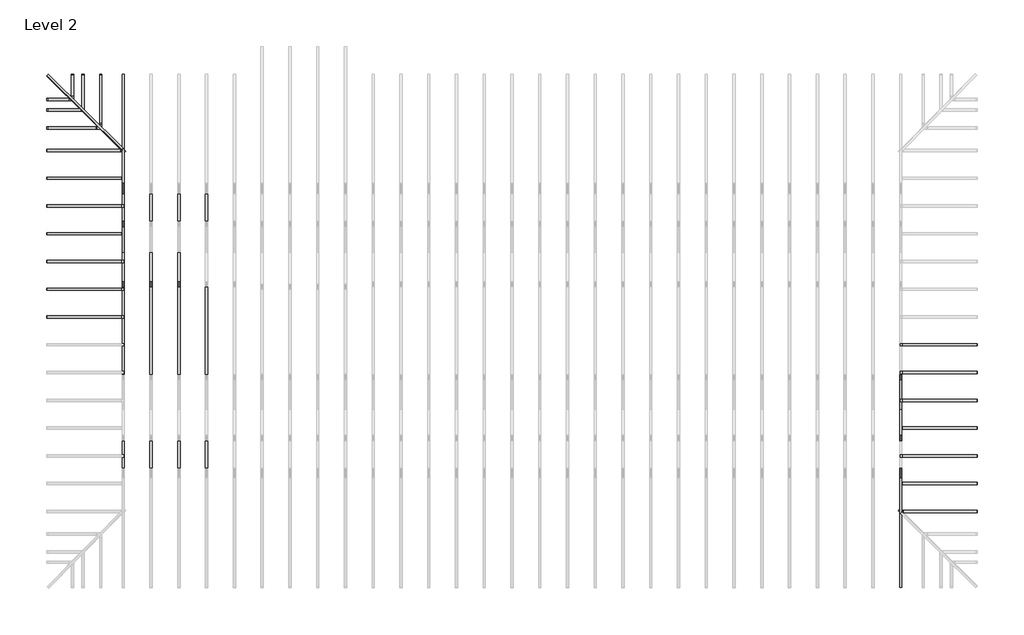
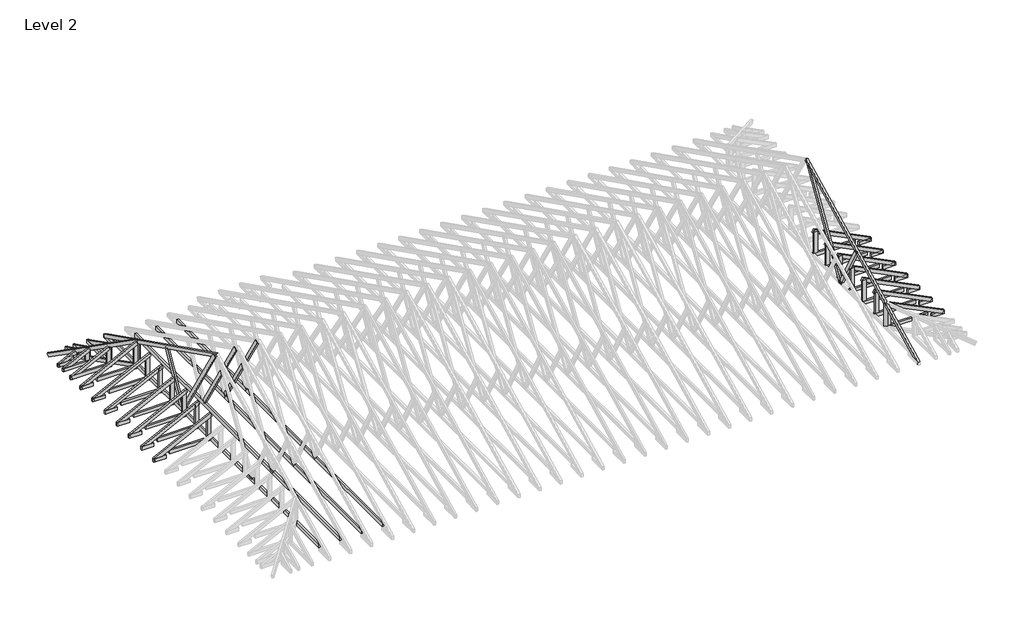
# One storey, part 3 of 5: 91 beams.
"""IFC4 building model written with IfcOpenShell, lengths in millimetres."""

import ifcopenshell
import ifcopenshell.guid

model = None  # the IFC model being written
_history = None  # IfcOwnerHistory: only IFC2X3 demands one
_inside = {}  # id of a spatial element -> (the spatial element, [elements in it])
_under = {}  # id of a project, library or spatial element -> (it, [spatial elements below it])
_declared = {}  # id of a project -> (the project, [libraries it declares])
_typed = {}  # id of a type object -> (the type object, [elements of that type])
_made_of = {}  # id of a material, layer set ... -> (it, [elements and type objects made of it])


def new_model(schema):
    """Start an empty IFC model of exactly this schema.

    Asked for "IFC4X3", IfcOpenShell would pick the latest addendum, in which some entities
    have other attributes; the version numbers below select the first issue.
    IFC2X3 requires an IfcOwnerHistory on every rooted entity: one is made here for all.
    """
    global model, _history
    if schema == "IFC4X3":
        model = ifcopenshell.file(schema_version=(4, 3, 0, 0))
    else:
        model = ifcopenshell.file(schema=schema)
    _inside.clear()
    _under.clear()
    _declared.clear()
    _typed.clear()
    _made_of.clear()
    _history = None
    if model.schema == "IFC2X3":
        org = make("IfcOrganization", Name="unknown")
        user = make(
            "IfcPersonAndOrganization",
            ThePerson=make("IfcPerson", FamilyName="unknown"),
            TheOrganization=org,
        )
        app = make(
            "IfcApplication",
            ApplicationDeveloper=org,
            Version="unknown",
            ApplicationFullName="unknown",
            ApplicationIdentifier="unknown",
        )
        _history = make(
            "IfcOwnerHistory",
            OwningUser=user,
            OwningApplication=app,
            ChangeAction="ADDED",
            CreationDate=0,
        )
    return model


def make(cls, **values):
    """One entity of the class cls with the attributes given. An attribute that is None is left unset."""
    return model.create_entity(
        cls, **{name: value for name, value in values.items() if value is not None}
    )


def rooted(cls, **values):
    """An entity with a GlobalId (a new one), such as an element, a storey or a relation."""
    return make(cls, GlobalId=ifcopenshell.guid.new(), OwnerHistory=_history, **values)


def si_unit(unit_type, name, prefix=None):
    """IfcSIUnit, for example si_unit("LENGTHUNIT", "METRE", prefix="MILLI")."""
    return make("IfcSIUnit", UnitType=unit_type, Prefix=prefix, Name=name)


def assignment(units):
    """IfcUnitAssignment: the units of a project."""
    return None if units is None else make("IfcUnitAssignment", Units=units)


def point(xyz):
    """IfcCartesianPoint."""
    return None if xyz is None else make("IfcCartesianPoint", Coordinates=xyz)


def direction(xyz):
    """IfcDirection."""
    return None if xyz is None else make("IfcDirection", DirectionRatios=xyz)


def frame(location, z_axis=None, x_axis=None):
    """IfcAxis2Placement3D, a coordinate frame: its origin and axes. An axis left out is left unset."""
    return make(
        "IfcAxis2Placement3D",
        Location=point(location),
        Axis=direction(z_axis),
        RefDirection=direction(x_axis),
    )


def origin():
    """The frame at (0, 0, 0) with its axes left unset."""
    return frame((0.0, 0.0, 0.0))


def place(relative_to, where):
    """IfcLocalPlacement: puts the frame where relative to a parent placement (None: the world)."""
    return make(
        "IfcLocalPlacement", PlacementRelTo=relative_to, RelativePlacement=where
    )


def context(
    kind, dimensions, precision=None, world=None, true_north=None, identifier=None
):
    """IfcGeometricRepresentationContext, for example the 3D "Model" context."""
    return make(
        "IfcGeometricRepresentationContext",
        ContextIdentifier=identifier,
        ContextType=kind,
        CoordinateSpaceDimension=dimensions,
        Precision=precision,
        WorldCoordinateSystem=world,
        TrueNorth=true_north,
    )


def project(units=None, contexts=None):
    """IfcProject with its units and contexts."""
    return rooted(
        "IfcProject",
        Name="project",
        RepresentationContexts=contexts,
        UnitsInContext=assignment(units),
    )


def spatial(cls, under=None, at=None, **own):
    """A site, building, storey or space (cls), placed at a placement, below another one or the project."""
    s = rooted(cls, ObjectPlacement=at, **own)
    if under is not None:
        _under.setdefault(under.id(), (under, []))[1].append(s)
    return s


def polyline(points):
    """IfcPolyline through the points."""
    return make("IfcPolyline", Points=[point(p) for p in points])


def outline(outer, holes=None, kind="AREA"):
    """IfcArbitraryClosedProfileDef: a profile drawn as a closed curve; with holes, ...WithVoids."""
    if holes is None:
        return make("IfcArbitraryClosedProfileDef", ProfileType=kind, OuterCurve=outer)
    return make(
        "IfcArbitraryProfileDefWithVoids",
        ProfileType=kind,
        OuterCurve=outer,
        InnerCurves=holes,
    )


def extrude(swept, where, along, depth):
    """IfcExtrudedAreaSolid: the profile swept, set in the frame where, extruded along a direction by depth."""
    return make(
        "IfcExtrudedAreaSolid",
        SweptArea=swept,
        Position=where,
        ExtrudedDirection=direction(along),
        Depth=depth,
    )


def shape(context_of_items, identifier, shape_type, items):
    """IfcShapeRepresentation: the items that make up one representation, for example the "Body"."""
    return make(
        "IfcShapeRepresentation",
        ContextOfItems=context_of_items,
        RepresentationIdentifier=identifier,
        RepresentationType=shape_type,
        Items=items,
    )


def source(mapping_origin, context_of_items, identifier, shape_type, items):
    """IfcRepresentationMap: a shape defined once, which mapped items show again and again."""
    return make(
        "IfcRepresentationMap",
        MappingOrigin=mapping_origin,
        MappedRepresentation=shape(context_of_items, identifier, shape_type, items),
    )


def transform(
    local_origin,
    x_axis=None,
    y_axis=None,
    z_axis=None,
    scale=None,
    scale2=None,
    scale3=None,
    uniform=True,
):
    """IfcCartesianTransformationOperator3D, or its non-uniform kind. x_axis, y_axis, z_axis: its Axis1, 2, 3."""
    if uniform:
        return make(
            "IfcCartesianTransformationOperator3D",
            Axis1=direction(x_axis),
            Axis2=direction(y_axis),
            LocalOrigin=point(local_origin),
            Scale=scale,
            Axis3=direction(z_axis),
        )
    return make(
        "IfcCartesianTransformationOperator3DnonUniform",
        Axis1=direction(x_axis),
        Axis2=direction(y_axis),
        LocalOrigin=point(local_origin),
        Scale=scale,
        Axis3=direction(z_axis),
        Scale2=scale2,
        Scale3=scale3,
    )


def mapped(mapping_source, mapping_target):
    """IfcMappedItem: shows the shape of a source again, moved by a transform."""
    return make(
        "IfcMappedItem", MappingSource=mapping_source, MappingTarget=mapping_target
    )


def made_of(thing, what):
    """Note that an element or type object is made of a material, layer set ...; save() writes the relation."""
    if what is not None:
        _made_of.setdefault(what.id(), (what, []))[1].append(thing)
    return thing


def element(
    cls,
    number,
    at=None,
    inside=None,
    cuts=None,
    type_object=None,
    material=None,
    context=None,
    identifier="Body",
    shape_type=None,
    held_by="IfcProductDefinitionShape",
    body=None,
    shapes=None,
    **own,
):
    """One element of the class cls, such as IfcWall. Its Tag is "e" and its number.

    at: its placement. inside: the storey or other place that contains it. cuts: it is an
    opening in that element (IfcRelVoidsElement). A single representation is given by context,
    identifier, shape_type and body (its items); several are given by shapes. held_by: the class
    of the entity that holds the representations. save() writes the other relations.
    """
    e = rooted(cls, Tag="e%d" % number, ObjectPlacement=at, **own)
    if body is not None:
        shapes = [shape(context, identifier, shape_type, body)]
    if shapes is not None:
        e.Representation = make(held_by, Representations=shapes)
    if inside is not None:
        _inside.setdefault(inside.id(), (inside, []))[1].append(e)
    if cuts is not None:
        rooted(
            "IfcRelVoidsElement", RelatingBuildingElement=cuts, RelatedOpeningElement=e
        )
    if type_object is not None:
        _typed.setdefault(type_object.id(), (type_object, []))[1].append(e)
    return made_of(e, material)


def aggregate(whole, parts):
    """IfcRelAggregates: a whole, such as a stair, and the parts it consists of."""
    return rooted("IfcRelAggregates", RelatingObject=whole, RelatedObjects=parts)


def save(model, path):
    """Write the relations noted so far, then the file.

    IfcRelAggregates (storeys below a building ...), IfcRelContainedInSpatialStructure (elements
    in a storey), IfcRelDefinesByType, IfcRelAssociatesMaterial and IfcRelDeclares: one each for
    every whole, place, type object, material and project.
    """
    for whole, parts in _under.values():
        aggregate(whole, parts)
    for where, things in _inside.values():
        rooted(
            "IfcRelContainedInSpatialStructure",
            RelatedElements=things,
            RelatingStructure=where,
        )
    for kind, things in _typed.values():
        rooted("IfcRelDefinesByType", RelatedObjects=things, RelatingType=kind)
    for what, things in _made_of.values():
        rooted("IfcRelAssociatesMaterial", RelatedObjects=things, RelatingMaterial=what)
    for by, libraries in _declared.values():
        rooted("IfcRelDeclares", RelatingContext=by, RelatedDefinitions=libraries)
    model.write(path)


def beam_90e8f76c(model_context):
    return source(origin(), model_context, "Body", "SweptSolid", [
        extrude(outline(polyline([(307.975, 25.4), (307.975, -25.4), (-47.625, -25.4), (-47.625, 25.4), (307.975, 25.4)])), frame((0.0, 0.0, -50.8), z_axis=(0.0, 0.0, 1.0), x_axis=(1.0, 0.0, 0.0)), (0.0, 0.0, 1.0), 101.6),
    ])


def beam_3a1eac92(model_context):
    return source(origin(), model_context, "Body", "SweptSolid", [
        extrude(outline(polyline([(233.4866591, 25.4), (233.4866591, -25.4), (-1464.867127, -25.4), (-1464.867127, 25.4), (233.4866591, 25.4)])), frame((0.0, 0.0, -50.8), z_axis=(0.0, 0.0, 1.0), x_axis=(1.0, 0.0, 0.0)), (0.0, 0.0, 1.0), 101.6),
    ])


def beam_38027485(model_context):
    return source(origin(), model_context, "Body", "SweptSolid", [
        extrude(outline(polyline([(595.8662636, 25.4), (595.8662636, -25.4), (-609.6, -25.4), (-609.6, 25.4), (595.8662636, 25.4)])), frame((0.0, 0.0, -50.8), z_axis=(0.0, 0.0, 1.0), x_axis=(1.0, 0.0, 0.0)), (0.0, 0.0, 1.0), 101.6),
    ])


def beam_7745fe0f(model_context):
    return source(origin(), model_context, "Body", "SweptSolid", [
        extrude(outline(polyline([(393.7, 25.4), (393.7, -25.4), (-393.7, -25.4), (-393.7, 25.4), (393.7, 25.4)])), frame((0.0, 0.0, -50.8), z_axis=(0.0, 0.0, 1.0), x_axis=(1.0, 0.0, 0.0)), (0.0, 0.0, 1.0), 101.6),
    ])


def beam_54dd7b45(model_context):
    return source(origin(), model_context, "Body", "SweptSolid", [
        extrude(outline(polyline([(393.7, -25.4), (-368.3, -25.4), (-368.3, 25.4), (393.7, 25.4), (393.7, -25.4)])), frame((0.0, 0.0, -50.8), z_axis=(0.0, 0.0, 1.0), x_axis=(1.0, 0.0, 0.0)), (0.0, 0.0, 1.0), 101.6),
    ])


def beam_85682148(model_context):
    return source(origin(), model_context, "Body", "SweptSolid", [
        extrude(outline(polyline([(595.8662636, -25.4), (-609.6, -25.4), (-609.6, 25.4), (595.8662636, 25.4), (595.8662636, -25.4)])), frame((0.0, 0.0, -50.8), z_axis=(0.0, 0.0, 1.0), x_axis=(1.0, 0.0, 0.0)), (0.0, 0.0, 1.0), 101.6),
    ])


def beam_154fe962(model_context):
    return source(origin(), model_context, "Body", "SweptSolid", [
        extrude(outline(polyline([(228.5999994, 25.4), (228.5999994, -25.4), (-228.6, -25.4), (-228.6, 25.4), (228.5999994, 25.4)])), frame((0.0, 0.0, -50.8), z_axis=(0.0, 0.0, 1.0), x_axis=(1.0, 0.0, 0.0)), (0.0, 0.0, 1.0), 101.6),
    ])


def beam_90eea034(model_context):
    return source(origin(), model_context, "Body", "SweptSolid", [
        extrude(outline(polyline([(821.193698, 25.4), (821.193698, -25.4), (-819.5010489, -25.4), (-819.5010489, 25.4), (821.193698, 25.4)])), frame((0.0, 0.0, -50.8), z_axis=(0.0, 0.0, 1.0), x_axis=(1.0, 0.0, 0.0)), (0.0, 0.0, 1.0), 101.6),
    ])


def beam_a4242642(model_context):
    return source(origin(), model_context, "Body", "SweptSolid", [
        extrude(outline(polyline([(5145.3336481, 25.4), (5145.3336481, -25.4), (-5145.3336481, -25.4), (-5145.3336481, 25.4), (5145.3336481, 25.4)])), frame((0.0, 0.0, -50.8), z_axis=(0.0, 0.0, 1.0), x_axis=(1.0, 0.0, 0.0)), (0.0, 0.0, 1.0), 101.6),
    ])


def beam_16181373(model_context):
    return source(origin(), model_context, "Body", "SweptSolid", [
        extrude(outline(polyline([(819.5010489, 25.4), (819.5010489, -25.4), (-821.193698, -25.4), (-821.193698, 25.4), (819.5010489, 25.4)])), frame((0.0, 0.0, -50.8), z_axis=(0.0, 0.0, 1.0), x_axis=(1.0, 0.0, 0.0)), (0.0, 0.0, 1.0), 101.6),
    ])


def beam_fc8bf4ae(model_context):
    return source(origin(), model_context, "Body", "SweptSolid", [
        extrude(outline(polyline([(1562.6646551, 25.4), (1562.6646551, -25.4), (-1550.1468127, -25.4), (-1550.1468127, 25.4), (1562.6646551, 25.4)])), frame((0.0, 0.0, -50.8), z_axis=(0.0, 0.0, 1.0), x_axis=(1.0, 0.0, 0.0)), (0.0, 0.0, 1.0), 101.6),
    ])


def beam_e838d316(model_context):
    return source(origin(), model_context, "Body", "SweptSolid", [
        extrude(outline(polyline([(1561.1045551, 25.4), (1561.1045551, -25.4), (-1572.5300502, -25.4), (-1572.5300502, 25.4), (1561.1045551, 25.4)])), frame((0.0, 0.0, -50.8), z_axis=(0.0, 0.0, 1.0), x_axis=(1.0, 0.0, 0.0)), (0.0, 0.0, 1.0), 101.6),
    ])


def beam_9afb64f6(model_context):
    return source(origin(), model_context, "Body", "SweptSolid", [
        extrude(outline(polyline([(365.3019367, 25.4), (365.3019367, -25.4), (-314.5019367, -25.4), (-314.5019367, 25.4), (365.3019367, 25.4)])), frame((0.0, 0.0, -50.8), z_axis=(0.0, 0.0, 1.0), x_axis=(1.0, 0.0, 0.0)), (0.0, 0.0, 1.0), 101.6),
    ])


def beam_87710fdd(model_context):
    return source(origin(), model_context, "Body", "SweptSolid", [
        extrude(outline(polyline([(147.1272806, 25.4), (147.1272806, -25.4), (-142.875, -25.4), (-142.875, 25.4), (147.1272806, 25.4)])), frame((0.0, 0.0, -50.8), z_axis=(0.0, 0.0, 1.0), x_axis=(1.0, 0.0, 0.0)), (0.0, 0.0, 1.0), 101.6),
    ])


def beam_29c6d41d(model_context):
    return source(origin(), model_context, "Body", "SweptSolid", [
        extrude(outline(polyline([(350.5042173, 25.4), (350.5042173, -25.4), (-295.4519367, -25.4), (-295.4519367, 25.4), (350.5042173, 25.4)])), frame((0.0, 0.0, -50.8), z_axis=(0.0, 0.0, 1.0), x_axis=(1.0, 0.0, 0.0)), (0.0, 0.0, 1.0), 101.6),
    ])


def beam_af5d22dc(model_context):
    return source(origin(), model_context, "Body", "SweptSolid", [
        extrude(outline(polyline([(571.5, 25.4), (571.5, -25.4), (-609.6, -25.4), (-609.6, 25.4), (571.5, 25.4)])), frame((0.0, 0.0, -50.8), z_axis=(0.0, 0.0, 1.0), x_axis=(1.0, 0.0, 0.0)), (0.0, 0.0, 1.0), 101.6),
    ])


def beam_7b8fa6d1(model_context):
    return source(origin(), model_context, "Body", "SweptSolid", [
        extrude(outline(polyline([(270.7395597, 25.4), (270.7395597, -25.4), (-219.9395597, -25.4), (-219.9395597, 25.4), (270.7395597, 25.4)])), frame((0.0, 0.0, -50.8), z_axis=(0.0, 0.0, 1.0), x_axis=(1.0, 0.0, 0.0)), (0.0, 0.0, 1.0), 101.6),
    ])


def beam_5e172d94(model_context):
    return source(origin(), model_context, "Body", "SweptSolid", [
        extrude(outline(polyline([(595.8662636, 25.4), (595.8662636, -25.4), (-548.2789755, -25.4), (-548.2789755, 25.4), (595.8662636, 25.4)])), frame((0.0, 0.0, -50.8), z_axis=(0.0, 0.0, 1.0), x_axis=(1.0, 0.0, 0.0)), (0.0, 0.0, 1.0), 101.6),
    ])


def beam_42a29ae5(model_context):
    return source(origin(), model_context, "Body", "SweptSolid", [
        extrude(outline(polyline([(270.7395597, -25.4), (-219.9395597, -25.4), (-219.9395597, 25.4), (270.7395597, 25.4), (270.7395597, -25.4)])), frame((0.0, 0.0, -50.8), z_axis=(0.0, 0.0, 1.0), x_axis=(1.0, 0.0, 0.0)), (0.0, 0.0, 1.0), 101.6),
    ])


def beam_11c5b8ca(model_context):
    return source(origin(), model_context, "Body", "SweptSolid", [
        extrude(outline(polyline([(147.1272806, -25.4), (-142.875, -25.4), (-142.875, 25.4), (147.1272806, 25.4), (147.1272806, -25.4)])), frame((0.0, 0.0, -50.8), z_axis=(0.0, 0.0, 1.0), x_axis=(1.0, 0.0, 0.0)), (0.0, 0.0, 1.0), 101.6),
    ])


def beam_5ac0b85f(model_context):
    return source(origin(), model_context, "Body", "SweptSolid", [
        extrude(outline(polyline([(571.5, -25.4), (-584.2, -25.4), (-584.2, 25.4), (571.5, 25.4), (571.5, -25.4)])), frame((0.0, 0.0, -50.8), z_axis=(0.0, 0.0, 1.0), x_axis=(1.0, 0.0, 0.0)), (0.0, 0.0, 1.0), 101.6),
    ])


def beam_99e5442a(model_context):
    return source(origin(), model_context, "Body", "SweptSolid", [
        extrude(outline(polyline([(350.5042173, -25.4), (-295.4519367, -25.4), (-295.4519367, 25.4), (350.5042173, 25.4), (350.5042173, -25.4)])), frame((0.0, 0.0, -50.8), z_axis=(0.0, 0.0, 1.0), x_axis=(1.0, 0.0, 0.0)), (0.0, 0.0, 1.0), 101.6),
    ])


def beam_38e3f9e5(model_context):
    return source(origin(), model_context, "Body", "SweptSolid", [
        extrude(outline(polyline([(595.8662636, -25.4), (-548.2789755, -25.4), (-548.2789755, 25.4), (595.8662636, 25.4), (595.8662636, -25.4)])), frame((0.0, 0.0, -50.8), z_axis=(0.0, 0.0, 1.0), x_axis=(1.0, 0.0, 0.0)), (0.0, 0.0, 1.0), 101.6),
    ])


def beam_7aad778a(model_context):
    return source(origin(), model_context, "Body", "SweptSolid", [
        extrude(outline(polyline([(307.975, -25.4), (-47.625, -25.4), (-47.625, 25.4), (307.975, 25.4), (307.975, -25.4)])), frame((0.0, 0.0, -50.8), z_axis=(0.0, 0.0, 1.0), x_axis=(1.0, 0.0, 0.0)), (0.0, 0.0, 1.0), 101.6),
    ])


def beam_878446a4(model_context):
    return source(origin(), model_context, "Body", "SweptSolid", [
        extrude(outline(polyline([(63.8057136, 25.4), (63.8057136, -25.4), (-59.553433, -25.4), (-59.553433, 25.4), (63.8057136, 25.4)])), frame((0.0, 0.0, -50.8), z_axis=(0.0, 0.0, 1.0), x_axis=(1.0, 0.0, 0.0)), (0.0, 0.0, 1.0), 101.6),
    ])


def beam_bc99fd75(model_context):
    return source(origin(), model_context, "Body", "SweptSolid", [
        extrude(outline(polyline([(222.3387319, 25.4), (222.3387319, -25.4), (-231.775, -25.4), (-231.775, 25.4), (222.3387319, 25.4)])), frame((0.0, 0.0, -50.8), z_axis=(0.0, 0.0, 1.0), x_axis=(1.0, 0.0, 0.0)), (0.0, 0.0, 1.0), 101.6),
    ])


def beam_efe25585(model_context):
    return source(origin(), model_context, "Body", "SweptSolid", [
        extrude(outline(polyline([(222.3387319, -25.4), (-231.775, -25.4), (-231.775, 25.4), (222.3387319, 25.4), (222.3387319, -25.4)])), frame((0.0, 0.0, -50.8), z_axis=(0.0, 0.0, 1.0), x_axis=(1.0, 0.0, 0.0)), (0.0, 0.0, 1.0), 101.6),
    ])


def beam_dfed05dc(model_context):
    return source(origin(), model_context, "Body", "SweptSolid", [
        extrude(outline(polyline([(63.8057136, -25.4), (-59.553433, -25.4), (-59.553433, 25.4), (63.8057136, 25.4), (63.8057136, -25.4)])), frame((0.0, 0.0, -50.8), z_axis=(0.0, 0.0, 1.0), x_axis=(1.0, 0.0, 0.0)), (0.0, 0.0, 1.0), 101.6),
    ])


model = new_model("IFC4")

# Units and contexts
model_context = context("Model", 3, world=origin())
ifc_project = project(units=[si_unit("LENGTHUNIT", "METRE", prefix="MILLI")], contexts=[model_context])

# Site, building, storey
site = spatial("IfcSite", under=ifc_project)
building = spatial("IfcBuilding", under=site)
storey = spatial("IfcBuildingStorey", under=building, Name="Level 2", Elevation=2768.6)

# Beams
placement = place(None, origin())
element("IfcBeam", 1, ObjectType="Dimension Lumber : BLDG 6241 2X4\" TRUSS MEMBER", at=placement, inside=storey, context=model_context, shape_type="SweptSolid", body=[
    extrude(outline(polyline([(0.0, -50.8), (0.0, 0.0), (6302.2496334, 0.0), (6302.2496334, -50.8), (0.0, -50.8)])), frame((-16607.414829, -17.2791662, 5496.1115355), z_axis=(0.0, 0.447213595499958, 0.894427190999916), x_axis=(0.0, 0.894427190999916, -0.447213595499958)), (0.0, 0.0, 1.0), 101.6),
])
element("IfcBeam", 2, ObjectType="Dimension Lumber : BLDG 6241 2X4\" TRUSS MEMBER", at=placement, inside=storey, context=model_context, shape_type="SweptSolid", body=[
    extrude(outline(polyline([(0.0, -50.8), (0.0, 0.0), (1828.8, 0.0), (1828.8, -50.8), (0.0, -50.8)])), frame((-18206.2149687, 3404.3284114, 2681.1076769), z_axis=(-0.44721359549995937, 0.0, 0.8944271909999152), x_axis=(0.8944271909999152, 0.0, 0.44721359549995937)), (0.0, 0.0, 1.0), 101.6),
])
element("IfcBeam", 3, ObjectType="Dimension Lumber : BLDG 6241 2X4\" TRUSS MEMBER", at=placement, inside=storey, context=model_context, shape_type="SweptSolid", body=[
    extrude(outline(polyline([(1e-07, -50.8), (0.0, 0.0), (2461.528697, 0.0), (2461.528697, -50.8), (1e-07, -50.8)])), frame((-16592.3107327, 3976.1580779, 3516.9362486), z_axis=(-0.2218309319850432, 0.2532052771584921, 0.9416358772018717), x_axis=(-0.6716162760239249, 0.6604274920267121, -0.33580813801196385)), (0.0, 0.0, 1.0), 101.6),
])
element("IfcBeam", 4, ObjectType="Dimension Lumber : BLDG 6241 2X4\" TRUSS MEMBER", at=placement, inside=storey, context=model_context, shape_type="SweptSolid", body=[
    extrude(outline(polyline([(0.0, -50.8), (0.0, 0.0), (1203.6219076, 0.0), (1203.6219076, -50.8), (0.0, -50.8)])), frame((-18207.7449824, 4509.2284114, 2680.3426701), z_axis=(-0.44721359549995937, 0.0, 0.8944271909999152), x_axis=(0.8944271909999152, 0.0, 0.44721359549995937)), (0.0, 0.0, 1.0), 101.6),
])
element("IfcBeam", 5, ObjectType="Dimension Lumber : BLDG 6241 2X4\" TRUSS MEMBER", at=placement, inside=storey, context=model_context, shape_type="SweptSolid", body=[
    extrude(outline(polyline([(0.0, -50.8), (0.0, 0.0), (844.55, 0.0), (844.55, -50.8), (0.0, -50.8)])), frame((-18212.4885612, 4902.9284114, 2677.9708807), z_axis=(-0.4472135954999599, 0.0, 0.894427190999915), x_axis=(0.894427190999915, 0.0, 0.4472135954999599)), (0.0, 0.0, 1.0), 101.6),
])
element("IfcBeam", 6, ObjectType="Dimension Lumber : BLDG 6241 2X4\" TRUSS MEMBER", at=placement, inside=storey, context=model_context, shape_type="SweptSolid", body=[
    extrude(outline(polyline([(0.0, -50.8), (0.0, 0.0), (6302.3539791, 0.0), (6302.3539791, -50.8), (0.0, -50.8)])), frame((461.385171, -5565.5155384, 2678.5857718), z_axis=(0.0, -0.447213595499958, 0.894427190999916), x_axis=(0.0, 0.894427190999916, 0.447213595499958)), (0.0, 0.0, 1.0), 101.6),
])
element("IfcBeam", 7, ObjectType="Dimension Lumber : BLDG 6241 2X4\" TRUSS MEMBER", at=placement, inside=storey, context=model_context, shape_type="SweptSolid", body=[
    extrude(outline(polyline([(0.0, -50.8), (0.0, 0.0), (1787.5128974, 0.0), (1787.5128974, -50.8), (0.0, -50.8)])), frame((-18206.2149687, 4013.9284114, 2681.1076769), z_axis=(-0.44721359549995937, 0.0, 0.8944271909999152), x_axis=(0.8944271909999152, 0.0, 0.44721359549995937)), (0.0, 0.0, 1.0), 101.6),
])
element("IfcBeam", 8, ObjectType="Dimension Lumber : BLDG 6241 2X4\" TRUSS MEMBER", at=placement, inside=storey, context=model_context, shape_type="SweptSolid", body=[
    extrude(outline(polyline([(0.0, -50.8), (0.0, 0.0), (1828.8, 0.0), (1828.8, -50.8), (0.0, -50.8)])), frame((-18206.2149687, 2794.7284114, 2681.1076769), z_axis=(-0.44721359549995937, 0.0, 0.8944271909999152), x_axis=(0.8944271909999152, 0.0, 0.44721359549995937)), (0.0, 0.0, 1.0), 101.6),
])
element("IfcBeam", 9, ObjectType="Dimension Lumber : BLDG 6241 2X4\" TRUSS MEMBER", at=placement, inside=storey, context=model_context, shape_type="SweptSolid", body=[
    extrude(outline(polyline([(0.0, -50.8), (0.0, 0.0), (1828.8, 0.0), (1828.8, -50.8), (0.0, -50.8)])), frame((-18206.2149687, 2185.1284114, 2681.1076769), z_axis=(-0.44721359549995937, 0.0, 0.8944271909999152), x_axis=(0.8944271909999152, 0.0, 0.44721359549995937)), (0.0, 0.0, 1.0), 101.6),
])
element("IfcBeam", 10, ObjectType="Dimension Lumber : BLDG 6241 2X4\" TRUSS MEMBER", at=placement, inside=storey, context=model_context, shape_type="SweptSolid", body=[
    extrude(outline(polyline([(0.0, -50.8), (0.0, 0.0), (1828.8, 0.0), (1828.8, -50.8), (0.0, -50.8)])), frame((-18206.2149687, 1575.5284114, 2681.1076769), z_axis=(-0.44721359549995937, 0.0, 0.8944271909999152), x_axis=(0.8944271909999152, 0.0, 0.44721359549995937)), (0.0, 0.0, 1.0), 101.6),
])
element("IfcBeam", 11, ObjectType="Dimension Lumber : BLDG 6241 2X4\" TRUSS MEMBER", at=placement, inside=storey, context=model_context, shape_type="SweptSolid", body=[
    extrude(outline(polyline([(0.0, -50.8), (0.0, 0.0), (1828.8, 0.0), (1828.8, -50.8), (0.0, -50.8)])), frame((-18206.2149687, 965.9284114, 2681.1076769), z_axis=(-0.44721359549995937, 0.0, 0.8944271909999152), x_axis=(0.8944271909999152, 0.0, 0.44721359549995937)), (0.0, 0.0, 1.0), 101.6),
])
element("IfcBeam", 12, ObjectType="Dimension Lumber : BLDG 6241 2X4\" TRUSS MEMBER", at=placement, inside=storey, context=model_context, shape_type="SweptSolid", body=[
    extrude(outline(polyline([(0.0, -50.8), (0.0, 0.0), (1828.8, 0.0), (1828.8, -50.8), (0.0, -50.8)])), frame((-18206.2149687, 356.3284114, 2681.1076769), z_axis=(-0.44721359549995937, 0.0, 0.8944271909999152), x_axis=(0.8944271909999152, 0.0, 0.44721359549995937)), (0.0, 0.0, 1.0), 101.6),
])
element("IfcBeam", 13, ObjectType="Dimension Lumber : BLDG 6241 2X4\" TRUSS MEMBER", at=placement, inside=storey, context=model_context, shape_type="SweptSolid", body=[
    extrude(outline(polyline([(0.0, 50.8), (1203.6219076, 50.8), (1203.6219076, 0.0), (0.0, 0.0), (0.0, 50.8)])), frame((-17102.714829, 5614.2585647, 2680.3426701), z_axis=(0.0, 0.44721359549995937, 0.8944271909999152), x_axis=(0.0, -0.8944271909999152, 0.44721359549995937)), (0.0, 0.0, 1.0), 101.6),
])
element("IfcBeam", 14, ObjectType="Dimension Lumber : BLDG 6241 2X4\" TRUSS MEMBER", at=placement, inside=storey, context=model_context, shape_type="SweptSolid", body=[
    extrude(outline(polyline([(0.0, 50.8), (844.55, 50.8), (844.55, 0.0), (0.0, 0.0), (0.0, 50.8)])), frame((-17496.414829, 5619.0021435, 2677.9708807), z_axis=(0.0, 0.4472135954999599, 0.894427190999915), x_axis=(0.0, -0.894427190999915, 0.4472135954999599)), (0.0, 0.0, 1.0), 101.6),
])
element("IfcBeam", 15, ObjectType="Dimension Lumber : BLDG 6241 2X4\" TRUSS MEMBER", at=placement, inside=storey, context=model_context, shape_type="SweptSolid", body=[
    extrude(outline(polyline([(0.0, 50.8), (1828.8, 50.8), (1828.8, 0.0), (0.0, 0.0), (0.0, 50.8)])), frame((2110.9853106, -253.2715886, 2681.1076769), z_axis=(0.44721359549995937, 0.0, 0.8944271909999152), x_axis=(-0.8944271909999152, 0.0, 0.44721359549995937)), (0.0, 0.0, 1.0), 101.6),
])
element("IfcBeam", 16, ObjectType="Dimension Lumber : BLDG 6241 2X4\" TRUSS MEMBER", at=placement, inside=storey, context=model_context, shape_type="SweptSolid", body=[
    extrude(outline(polyline([(0.0, 50.8), (1828.8, 50.8), (1828.8, 0.0), (0.0, 0.0), (0.0, 50.8)])), frame((2110.9853106, -862.8715886, 2681.1076769), z_axis=(0.44721359549995937, 0.0, 0.8944271909999152), x_axis=(-0.8944271909999152, 0.0, 0.44721359549995937)), (0.0, 0.0, 1.0), 101.6),
])
element("IfcBeam", 17, ObjectType="Dimension Lumber : BLDG 6241 2X4\" TRUSS MEMBER", at=placement, inside=storey, context=model_context, shape_type="SweptSolid", body=[
    extrude(outline(polyline([(0.0, 50.8), (1828.8, 50.8), (1828.8, 0.0), (0.0, 0.0), (0.0, 50.8)])), frame((2110.9853106, -1472.4715886, 2681.1076769), z_axis=(0.44721359549995937, 0.0, 0.8944271909999152), x_axis=(-0.8944271909999152, 0.0, 0.44721359549995937)), (0.0, 0.0, 1.0), 101.6),
])
element("IfcBeam", 18, ObjectType="Dimension Lumber : BLDG 6241 2X4\" TRUSS MEMBER", at=placement, inside=storey, context=model_context, shape_type="SweptSolid", body=[
    extrude(outline(polyline([(0.0, 50.8), (1828.8, 50.8), (1828.8, 0.0), (0.0, 0.0), (0.0, 50.8)])), frame((2110.9853106, -2082.0715886, 2681.1076769), z_axis=(0.44721359549995937, 0.0, 0.8944271909999152), x_axis=(-0.8944271909999152, 0.0, 0.44721359549995937)), (0.0, 0.0, 1.0), 101.6),
])
element("IfcBeam", 19, ObjectType="Dimension Lumber : BLDG 6241 2X4\" TRUSS MEMBER", at=placement, inside=storey, context=model_context, shape_type="SweptSolid", body=[
    extrude(outline(polyline([(0.0, 50.8), (1828.8, 50.8), (1828.8, 0.0), (0.0, 0.0), (0.0, 50.8)])), frame((2110.9853106, -2691.6715886, 2681.1076769), z_axis=(0.44721359549995937, 0.0, 0.8944271909999152), x_axis=(-0.8944271909999152, 0.0, 0.44721359549995937)), (0.0, 0.0, 1.0), 101.6),
])
element("IfcBeam", 20, ObjectType="Dimension Lumber : BLDG 6241 2X4\" TRUSS MEMBER", at=placement, inside=storey, context=model_context, shape_type="SweptSolid", body=[
    extrude(outline(polyline([(0.0, 50.8), (1828.8, 50.8), (1828.8, 0.0), (0.0, 0.0), (0.0, 50.8)])), frame((2110.9853106, -3301.2715886, 2681.1076769), z_axis=(0.44721359549995937, 0.0, 0.8944271909999152), x_axis=(-0.8944271909999152, 0.0, 0.44721359549995937)), (0.0, 0.0, 1.0), 101.6),
])
element("IfcBeam", 21, ObjectType="Dimension Lumber : BLDG 6241 2X4\" TRUSS MEMBER", at=placement, inside=storey, context=model_context, shape_type="SweptSolid", body=[
    extrude(outline(polyline([(0.0, 50.8), (1787.5128973, 50.8), (1787.5128973, 0.0), (0.0, 0.0), (0.0, 50.8)])), frame((2110.9853106, -3910.8715886, 2681.1076769), z_axis=(0.44721359549995937, 0.0, 0.8944271909999152), x_axis=(-0.8944271909999152, 0.0, 0.44721359549995937)), (0.0, 0.0, 1.0), 101.6),
])
element("IfcBeam", 22, ObjectType="Dimension Lumber : BLDG 6241 2X4\" TRUSS MEMBER", at=placement, inside=storey, context=model_context, shape_type="SweptSolid", body=[
    extrude(outline(polyline([(0.0, -50.8), (0.0, 0.0), (546.1, 0.0), (546.1, -50.8), (0.0, -50.8)])), frame((-18212.1757804, 5131.5284114, 2678.127271), z_axis=(-0.4472135954999593, 0.0, 0.8944271909999153), x_axis=(0.8944271909999153, 0.0, 0.4472135954999593)), (0.0, 0.0, 1.0), 101.6),
])
element("IfcBeam", 23, ObjectType="Dimension Lumber : BLDG 6241 2X4\" TRUSS MEMBER", at=placement, inside=storey, context=model_context, shape_type="SweptSolid", body=[
    extrude(outline(polyline([(0.0, 50.8), (546.1, 50.8), (546.1, 0.0), (0.0, 0.0), (0.0, 50.8)])), frame((-17725.014829, 5618.6893628, 2678.127271), z_axis=(0.0, 0.4472135954999592, 0.8944271909999153), x_axis=(0.0, -0.8944271909999153, 0.4472135954999592)), (0.0, 0.0, 1.0), 101.6),
])
beam_shape = beam_90e8f76c(model_context)
element("IfcBeam", 24, ObjectType="Dimension Lumber : BLDG 6241 2X4\" TRUSS MEMBER", at=placement, inside=storey, context=model_context, shape_type="MappedRepresentation", body=[
    mapped(beam_shape, transform((-18210.789829, 3378.9284114, 2717.8), x_axis=(1.0, 0.0, 0.0), y_axis=(0.0, 1.0, 0.0), z_axis=(0.0, 0.0, 1.0))),
])
element("IfcBeam", 25, ObjectType="Dimension Lumber : BLDG 6241 2X4\" TRUSS MEMBER", at=placement, inside=storey, context=model_context, shape_type="MappedRepresentation", body=[
    mapped(beam_shape, transform((-18210.789829, 3988.5284114, 2717.8), x_axis=(1.0, 0.0, 0.0), y_axis=(0.0, 1.0, 0.0), z_axis=(0.0, 0.0, 1.0))),
])
element("IfcBeam", 26, ObjectType="Dimension Lumber : BLDG 6241 2X4\" TRUSS MEMBER", at=placement, inside=storey, context=model_context, shape_type="MappedRepresentation", body=[
    mapped(beam_shape, transform((-18210.789829, 2769.3284114, 2717.8), x_axis=(1.0, 0.0, 0.0), y_axis=(0.0, 1.0, 0.0), z_axis=(0.0, 0.0, 1.0))),
])
element("IfcBeam", 27, ObjectType="Dimension Lumber : BLDG 6241 2X4\" TRUSS MEMBER", at=placement, inside=storey, context=model_context, shape_type="MappedRepresentation", body=[
    mapped(beam_shape, transform((-18210.789829, 2159.7284114, 2717.8), x_axis=(1.0, 0.0, 0.0), y_axis=(0.0, 1.0, 0.0), z_axis=(0.0, 0.0, 1.0))),
])
element("IfcBeam", 28, ObjectType="Dimension Lumber : BLDG 6241 2X4\" TRUSS MEMBER", at=placement, inside=storey, context=model_context, shape_type="MappedRepresentation", body=[
    mapped(beam_shape, transform((-18210.789829, 1550.1284114, 2717.8), x_axis=(1.0, 0.0, 0.0), y_axis=(0.0, 1.0, 0.0), z_axis=(0.0, 0.0, 1.0))),
])
element("IfcBeam", 29, ObjectType="Dimension Lumber : BLDG 6241 2X4\" TRUSS MEMBER", at=placement, inside=storey, context=model_context, shape_type="MappedRepresentation", body=[
    mapped(beam_shape, transform((-18210.789829, 940.5284114, 2717.8), x_axis=(1.0, 0.0, 0.0), y_axis=(0.0, 1.0, 0.0), z_axis=(0.0, 0.0, 1.0))),
])
element("IfcBeam", 30, ObjectType="Dimension Lumber : BLDG 6241 2X4\" TRUSS MEMBER", at=placement, inside=storey, context=model_context, shape_type="MappedRepresentation", body=[
    mapped(beam_shape, transform((-18210.789829, 330.9284114, 2717.8), x_axis=(1.0, 0.0, 0.0), y_axis=(0.0, 1.0, 0.0), z_axis=(0.0, 0.0, 1.0))),
])
beam_2_shape = beam_3a1eac92(model_context)
element("IfcBeam", 31, ObjectType="Dimension Lumber : BLDG 6241 2X4\" TRUSS MEMBER", at=placement, inside=storey, context=model_context, shape_type="MappedRepresentation", body=[
    mapped(beam_2_shape, transform((-16772.514829, 4179.0284114, 2819.4), x_axis=(0.7071067811865462, -0.7071067811865488, 0.0), y_axis=(0.7071067811865488, 0.7071067811865462, 0.0), z_axis=(0.0, 0.0, 1.0))),
])
beam_3_shape = beam_38027485(model_context)
element("IfcBeam", 32, ObjectType="Dimension Lumber : BLDG 6241 2X4\" TRUSS MEMBER", at=placement, inside=storey, context=model_context, shape_type="MappedRepresentation", body=[
    mapped(beam_3_shape, transform((-17191.614829, 3378.9284114, 2819.4), x_axis=(-1.0, 0.0, 0.0), y_axis=(0.0, -1.0, 0.0), z_axis=(0.0, 0.0, 1.0))),
])
element("IfcBeam", 33, ObjectType="Dimension Lumber : BLDG 6241 2X4\" TRUSS MEMBER", at=placement, inside=storey, context=model_context, shape_type="MappedRepresentation", body=[
    mapped(beam_3_shape, transform((-17191.614829, 2769.3284114, 2819.4), x_axis=(-1.0, 0.0, 0.0), y_axis=(0.0, -1.0, 0.0), z_axis=(0.0, 0.0, 1.0))),
])
element("IfcBeam", 34, ObjectType="Dimension Lumber : BLDG 6241 2X4\" TRUSS MEMBER", at=placement, inside=storey, context=model_context, shape_type="MappedRepresentation", body=[
    mapped(beam_3_shape, transform((-17191.614829, 2159.7284114, 2819.4), x_axis=(-1.0, 0.0, 0.0), y_axis=(0.0, -1.0, 0.0), z_axis=(0.0, 0.0, 1.0))),
])
element("IfcBeam", 35, ObjectType="Dimension Lumber : BLDG 6241 2X4\" TRUSS MEMBER", at=placement, inside=storey, context=model_context, shape_type="MappedRepresentation", body=[
    mapped(beam_3_shape, transform((-17191.614829, 1550.1284114, 2819.4), x_axis=(-1.0, 0.0, 0.0), y_axis=(0.0, -1.0, 0.0), z_axis=(0.0, 0.0, 1.0))),
])
element("IfcBeam", 36, ObjectType="Dimension Lumber : BLDG 6241 2X4\" TRUSS MEMBER", at=placement, inside=storey, context=model_context, shape_type="MappedRepresentation", body=[
    mapped(beam_3_shape, transform((-17191.614829, 940.5284114, 2819.4), x_axis=(-1.0, 0.0, 0.0), y_axis=(0.0, -1.0, 0.0), z_axis=(0.0, 0.0, 1.0))),
])
element("IfcBeam", 37, ObjectType="Dimension Lumber : BLDG 6241 2X4\" TRUSS MEMBER", at=placement, inside=storey, context=model_context, shape_type="MappedRepresentation", body=[
    mapped(beam_3_shape, transform((-17191.614829, 330.9284114, 2819.4), x_axis=(-1.0, 0.0, 0.0), y_axis=(0.0, -1.0, 0.0), z_axis=(0.0, 0.0, 1.0))),
])
beam_4_shape = beam_7745fe0f(model_context)
element("IfcBeam", 38, ObjectType="Dimension Lumber : BLDG 6241 2X4\" TRUSS MEMBER", at=placement, inside=storey, context=model_context, shape_type="MappedRepresentation", body=[
    mapped(beam_4_shape, transform((-17864.714829, 4877.5284114, 2728.7708807), x_axis=(-1.0, 0.0, 0.0), y_axis=(0.0, -1.0, 0.0), z_axis=(0.0, 0.0, 1.0))),
])
beam_5_shape = beam_54dd7b45(model_context)
element("IfcBeam", 39, ObjectType="Dimension Lumber : BLDG 6241 2X4\" TRUSS MEMBER", at=placement, inside=storey, context=model_context, shape_type="MappedRepresentation", body=[
    mapped(beam_5_shape, transform((-17471.014829, 5271.2284114, 2728.7708807), x_axis=(0.0, 1.0, 0.0), y_axis=(-1.0, 0.0, 0.0), z_axis=(0.0, 0.0, 1.0))),
])
beam_6_shape = beam_85682148(model_context)
element("IfcBeam", 40, ObjectType="Dimension Lumber : BLDG 6241 2X4\" TRUSS MEMBER", at=placement, inside=storey, context=model_context, shape_type="MappedRepresentation", body=[
    mapped(beam_6_shape, transform((1096.385171, -278.6715886, 2819.4), x_axis=(1.0, 0.0, 0.0), y_axis=(0.0, 1.0, 0.0), z_axis=(0.0, 0.0, 1.0))),
])
element("IfcBeam", 41, ObjectType="Dimension Lumber : BLDG 6241 2X4\" TRUSS MEMBER", at=placement, inside=storey, context=model_context, shape_type="MappedRepresentation", body=[
    mapped(beam_6_shape, transform((1096.385171, -888.2715886, 2819.4), x_axis=(1.0, 0.0, 0.0), y_axis=(0.0, 1.0, 0.0), z_axis=(0.0, 0.0, 1.0))),
])
element("IfcBeam", 42, ObjectType="Dimension Lumber : BLDG 6241 2X4\" TRUSS MEMBER", at=placement, inside=storey, context=model_context, shape_type="MappedRepresentation", body=[
    mapped(beam_6_shape, transform((1096.385171, -1497.8715886, 2819.4), x_axis=(1.0, 0.0, 0.0), y_axis=(0.0, 1.0, 0.0), z_axis=(0.0, 0.0, 1.0))),
])
element("IfcBeam", 43, ObjectType="Dimension Lumber : BLDG 6241 2X4\" TRUSS MEMBER", at=placement, inside=storey, context=model_context, shape_type="MappedRepresentation", body=[
    mapped(beam_6_shape, transform((1096.385171, -2107.4715886, 2819.4), x_axis=(1.0, 0.0, 0.0), y_axis=(0.0, 1.0, 0.0), z_axis=(0.0, 0.0, 1.0))),
])
element("IfcBeam", 44, ObjectType="Dimension Lumber : BLDG 6241 2X4\" TRUSS MEMBER", at=placement, inside=storey, context=model_context, shape_type="MappedRepresentation", body=[
    mapped(beam_6_shape, transform((1096.385171, -2717.0715886, 2819.4), x_axis=(1.0, 0.0, 0.0), y_axis=(0.0, 1.0, 0.0), z_axis=(0.0, 0.0, 1.0))),
])
element("IfcBeam", 45, ObjectType="Dimension Lumber : BLDG 6241 2X4\" TRUSS MEMBER", at=placement, inside=storey, context=model_context, shape_type="MappedRepresentation", body=[
    mapped(beam_6_shape, transform((1096.385171, -3326.6715886, 2819.4), x_axis=(1.0, 0.0, 0.0), y_axis=(0.0, 1.0, 0.0), z_axis=(0.0, 0.0, 1.0))),
])
beam_7_shape = beam_154fe962(model_context)
element("IfcBeam", 46, ObjectType="Dimension Lumber : BLDG 6241 2X4\" TRUSS MEMBER", at=placement, inside=storey, context=model_context, shape_type="MappedRepresentation", body=[
    mapped(beam_7_shape, transform((-16582.014829, 5436.3284114, 2717.8), x_axis=(0.0, -1.0, 0.0), y_axis=(1.0, 0.0, 0.0), z_axis=(0.0, 0.0, 1.0))),
])
beam_8_shape = beam_90eea034(model_context)
element("IfcBeam", 47, ObjectType="Dimension Lumber : BLDG 6241 2X4\" TRUSS MEMBER", at=placement, inside=storey, context=model_context, shape_type="MappedRepresentation", body=[
    mapped(beam_8_shape, transform((-16582.014829, 2147.8781861, 3552.5770493), x_axis=(0.0, -0.4803172630852001, -0.8770948220017848), y_axis=(-1.0, 0.0, 0.0), z_axis=(0.0, 0.8770948220017848, -0.4803172630852001))),
])
beam_9_shape = beam_a4242642(model_context)
element("IfcBeam", 48, ObjectType="Dimension Lumber : BLDG 6241 2X4\" TRUSS MEMBER", at=placement, inside=storey, context=model_context, shape_type="MappedRepresentation", body=[
    mapped(beam_9_shape, transform((-16582.014829, 26.1284114, 2819.4), x_axis=(0.0, -1.0, 0.0), y_axis=(1.0, 0.0, 0.0), z_axis=(0.0, 0.0, 1.0))),
])
element("IfcBeam", 49, ObjectType="Dimension Lumber : BLDG 6241 2X4\" TRUSS MEMBER", at=placement, inside=storey, context=model_context, shape_type="MappedRepresentation", body=[
    mapped(beam_9_shape, transform((-15972.414829, 26.1284114, 2819.4), x_axis=(0.0, -1.0, 0.0), y_axis=(1.0, 0.0, 0.0), z_axis=(0.0, 0.0, 1.0))),
])
element("IfcBeam", 50, ObjectType="Dimension Lumber : BLDG 6241 2X4\" TRUSS MEMBER", at=placement, inside=storey, context=model_context, shape_type="MappedRepresentation", body=[
    mapped(beam_9_shape, transform((-15362.814829, 26.1284114, 2819.4), x_axis=(0.0, -1.0, 0.0), y_axis=(1.0, 0.0, 0.0), z_axis=(0.0, 0.0, 1.0))),
])
element("IfcBeam", 51, ObjectType="Dimension Lumber : BLDG 6241 2X4\" TRUSS MEMBER", at=placement, inside=storey, context=model_context, shape_type="MappedRepresentation", body=[
    mapped(beam_9_shape, transform((-14753.214829, 26.1284114, 2819.4), x_axis=(0.0, -1.0, 0.0), y_axis=(1.0, 0.0, 0.0), z_axis=(0.0, 0.0, 1.0))),
])
beam_10_shape = beam_16181373(model_context)
element("IfcBeam", 52, ObjectType="Dimension Lumber : BLDG 6241 2X4\" TRUSS MEMBER", at=placement, inside=storey, context=model_context, shape_type="MappedRepresentation", body=[
    mapped(beam_10_shape, transform((486.785171, -2095.6213634, 3552.5770493), x_axis=(0.0, -0.4803172630852174, 0.8770948220017754), y_axis=(-1.0, 0.0, 0.0), z_axis=(0.0, -0.8770948220017754, -0.4803172630852174))),
])
beam_11_shape = beam_fc8bf4ae(model_context)
element("IfcBeam", 53, ObjectType="Dimension Lumber : BLDG 6241 2X4\" TRUSS MEMBER", at=placement, inside=storey, context=model_context, shape_type="MappedRepresentation", body=[
    mapped(beam_11_shape, transform((-16582.014829, 944.3448606, 4154.3437121), x_axis=(0.0, -0.5218941539815979, 0.8530102531856415), y_axis=(-1.0, 0.0, 0.0), z_axis=(0.0, -0.8530102531856415, -0.5218941539815979))),
])
element("IfcBeam", 54, ObjectType="Dimension Lumber : BLDG 6241 2X4\" TRUSS MEMBER", at=placement, inside=storey, context=model_context, shape_type="MappedRepresentation", body=[
    mapped(beam_11_shape, transform((-15972.414829, 944.3448606, 4154.3437121), x_axis=(0.0, -0.5218941539815979, 0.8530102531856415), y_axis=(-1.0, 0.0, 0.0), z_axis=(0.0, -0.8530102531856415, -0.5218941539815979))),
])
element("IfcBeam", 55, ObjectType="Dimension Lumber : BLDG 6241 2X4\" TRUSS MEMBER", at=placement, inside=storey, context=model_context, shape_type="MappedRepresentation", body=[
    mapped(beam_11_shape, transform((-15362.814829, 944.3448606, 4154.3437121), x_axis=(0.0, -0.5218941539815979, 0.8530102531856415), y_axis=(-1.0, 0.0, 0.0), z_axis=(0.0, -0.8530102531856415, -0.5218941539815979))),
])
beam_12_shape = beam_e838d316(model_context)
element("IfcBeam", 56, ObjectType="Dimension Lumber : BLDG 6241 2X4\" TRUSS MEMBER", at=placement, inside=storey, context=model_context, shape_type="MappedRepresentation", body=[
    mapped(beam_12_shape, transform((486.785171, -880.0831247, 4160.3461686), x_axis=(0.0, -0.5257715142502325, -0.8506258371358218), y_axis=(-1.0, 0.0, 0.0), z_axis=(0.0, 0.8506258371358218, -0.5257715142502325))),
])
beam_13_shape = beam_9afb64f6(model_context)
element("IfcBeam", 57, ObjectType="Dimension Lumber : BLDG 6241 2X4\" TRUSS MEMBER", at=placement, inside=storey, context=model_context, shape_type="MappedRepresentation", body=[
    mapped(beam_13_shape, transform((-16582.014829, 3988.5284114, 3184.7019367), x_axis=(0.0, 0.0, 1.0), y_axis=(-0.7071067811865501, -0.7071067811865449, 0.0), z_axis=(0.7071067811865449, -0.7071067811865501, 0.0))),
])
element("IfcBeam", 58, ObjectType="Dimension Lumber : BLDG 6241 2X4\" TRUSS MEMBER", at=placement, inside=storey, context=model_context, shape_type="MappedRepresentation", body=[
    mapped(beam_13_shape, transform((486.785171, -3936.2715886, 3184.7019367), x_axis=(0.0, 0.0, 1.0), y_axis=(0.7071067811865456, 0.7071067811865495, 0.0), z_axis=(-0.7071067811865495, 0.7071067811865456, 0.0))),
])
beam_14_shape = beam_87710fdd(model_context)
element("IfcBeam", 59, ObjectType="Dimension Lumber : BLDG 6241 2X4\" TRUSS MEMBER", at=placement, inside=storey, context=model_context, shape_type="MappedRepresentation", body=[
    mapped(beam_14_shape, transform((-17547.214829, 4877.5284114, 2924.5288734), x_axis=(0.0, 0.0, 1.0), y_axis=(0.0, 1.0, 0.0), z_axis=(-1.0, 0.0, 0.0))),
])
beam_15_shape = beam_29c6d41d(model_context)
element("IfcBeam", 60, ObjectType="Dimension Lumber : BLDG 6241 2X4\" TRUSS MEMBER", at=placement, inside=storey, context=model_context, shape_type="MappedRepresentation", body=[
    mapped(beam_15_shape, transform((-16658.214829, 3378.9284114, 3165.6519367), x_axis=(0.0, 0.0, 1.0), y_axis=(0.0, 1.0, 0.0), z_axis=(-1.0, 0.0, 0.0))),
])
element("IfcBeam", 61, ObjectType="Dimension Lumber : BLDG 6241 2X4\" TRUSS MEMBER", at=placement, inside=storey, context=model_context, shape_type="MappedRepresentation", body=[
    mapped(beam_15_shape, transform((-16658.214829, 3988.5284114, 3165.6519367), x_axis=(0.0, 0.0, 1.0), y_axis=(0.0, 1.0, 0.0), z_axis=(-1.0, 0.0, 0.0))),
])
element("IfcBeam", 62, ObjectType="Dimension Lumber : BLDG 6241 2X4\" TRUSS MEMBER", at=placement, inside=storey, context=model_context, shape_type="MappedRepresentation", body=[
    mapped(beam_15_shape, transform((-16658.214829, 2769.3284114, 3165.6519367), x_axis=(0.0, 0.0, 1.0), y_axis=(0.0, 1.0, 0.0), z_axis=(-1.0, 0.0, 0.0))),
])
element("IfcBeam", 63, ObjectType="Dimension Lumber : BLDG 6241 2X4\" TRUSS MEMBER", at=placement, inside=storey, context=model_context, shape_type="MappedRepresentation", body=[
    mapped(beam_15_shape, transform((-16658.214829, 2159.7284114, 3165.6519367), x_axis=(0.0, 0.0, 1.0), y_axis=(0.0, 1.0, 0.0), z_axis=(-1.0, 0.0, 0.0))),
])
element("IfcBeam", 64, ObjectType="Dimension Lumber : BLDG 6241 2X4\" TRUSS MEMBER", at=placement, inside=storey, context=model_context, shape_type="MappedRepresentation", body=[
    mapped(beam_15_shape, transform((-16658.214829, 1550.1284114, 3165.6519367), x_axis=(0.0, 0.0, 1.0), y_axis=(0.0, 1.0, 0.0), z_axis=(-1.0, 0.0, 0.0))),
])
element("IfcBeam", 65, ObjectType="Dimension Lumber : BLDG 6241 2X4\" TRUSS MEMBER", at=placement, inside=storey, context=model_context, shape_type="MappedRepresentation", body=[
    mapped(beam_15_shape, transform((-16658.214829, 940.5284114, 3165.6519367), x_axis=(0.0, 0.0, 1.0), y_axis=(0.0, 1.0, 0.0), z_axis=(-1.0, 0.0, 0.0))),
])
element("IfcBeam", 66, ObjectType="Dimension Lumber : BLDG 6241 2X4\" TRUSS MEMBER", at=placement, inside=storey, context=model_context, shape_type="MappedRepresentation", body=[
    mapped(beam_15_shape, transform((-16658.214829, 330.9284114, 3165.6519367), x_axis=(0.0, 0.0, 1.0), y_axis=(0.0, 1.0, 0.0), z_axis=(-1.0, 0.0, 0.0))),
])
beam_16_shape = beam_af5d22dc(model_context)
element("IfcBeam", 67, ObjectType="Dimension Lumber : BLDG 6241 2X4\" TRUSS MEMBER", at=placement, inside=storey, context=model_context, shape_type="MappedRepresentation", body=[
    mapped(beam_16_shape, transform((-17686.914829, 4483.8284114, 2728.7708807), x_axis=(-1.0, 0.0, 0.0), y_axis=(0.0, -1.0, 0.0), z_axis=(0.0, 0.0, 1.0))),
])
beam_17_shape = beam_7b8fa6d1(model_context)
element("IfcBeam", 68, ObjectType="Dimension Lumber : BLDG 6241 2X4\" TRUSS MEMBER", at=placement, inside=storey, context=model_context, shape_type="MappedRepresentation", body=[
    mapped(beam_17_shape, transform((-17153.514829, 4483.8284114, 2999.5104403), x_axis=(0.0, 0.0, 1.0), y_axis=(0.0, 1.0, 0.0), z_axis=(-1.0, 0.0, 0.0))),
])
beam_18_shape = beam_5e172d94(model_context)
element("IfcBeam", 69, ObjectType="Dimension Lumber : BLDG 6241 2X4\" TRUSS MEMBER", at=placement, inside=storey, context=model_context, shape_type="MappedRepresentation", body=[
    mapped(beam_18_shape, transform((-17191.614829, 3988.5284114, 2819.4), x_axis=(-1.0, 0.0, 0.0), y_axis=(0.0, -1.0, 0.0), z_axis=(0.0, 0.0, 1.0))),
])
beam_19_shape = beam_42a29ae5(model_context)
element("IfcBeam", 70, ObjectType="Dimension Lumber : BLDG 6241 2X4\" TRUSS MEMBER", at=placement, inside=storey, context=model_context, shape_type="MappedRepresentation", body=[
    mapped(beam_19_shape, transform((-17077.314829, 4560.0284114, 2999.5104403), x_axis=(0.0, 0.0, 1.0), y_axis=(1.0, 0.0, 0.0), z_axis=(0.0, 1.0, 0.0))),
])
beam_20_shape = beam_11c5b8ca(model_context)
element("IfcBeam", 71, ObjectType="Dimension Lumber : BLDG 6241 2X4\" TRUSS MEMBER", at=placement, inside=storey, context=model_context, shape_type="MappedRepresentation", body=[
    mapped(beam_20_shape, transform((-17471.014829, 4953.7284114, 2924.5288734), x_axis=(0.0, 0.0, 1.0), y_axis=(1.0, 0.0, 0.0), z_axis=(0.0, 1.0, 0.0))),
])
beam_21_shape = beam_5ac0b85f(model_context)
element("IfcBeam", 72, ObjectType="Dimension Lumber : BLDG 6241 2X4\" TRUSS MEMBER", at=placement, inside=storey, context=model_context, shape_type="MappedRepresentation", body=[
    mapped(beam_21_shape, transform((-17077.314829, 5093.4284114, 2728.7708807), x_axis=(0.0, 1.0, 0.0), y_axis=(-1.0, 0.0, 0.0), z_axis=(0.0, 0.0, 1.0))),
])
beam_22_shape = beam_99e5442a(model_context)
element("IfcBeam", 73, ObjectType="Dimension Lumber : BLDG 6241 2X4\" TRUSS MEMBER", at=placement, inside=storey, context=model_context, shape_type="MappedRepresentation", body=[
    mapped(beam_22_shape, transform((562.985171, -278.6715886, 3165.6519367), x_axis=(0.0, 0.0, 1.0), y_axis=(0.0, -1.0, 0.0), z_axis=(1.0, 0.0, 0.0))),
])
element("IfcBeam", 74, ObjectType="Dimension Lumber : BLDG 6241 2X4\" TRUSS MEMBER", at=placement, inside=storey, context=model_context, shape_type="MappedRepresentation", body=[
    mapped(beam_22_shape, transform((562.985171, -888.2715886, 3165.6519367), x_axis=(0.0, 0.0, 1.0), y_axis=(0.0, -1.0, 0.0), z_axis=(1.0, 0.0, 0.0))),
])
element("IfcBeam", 75, ObjectType="Dimension Lumber : BLDG 6241 2X4\" TRUSS MEMBER", at=placement, inside=storey, context=model_context, shape_type="MappedRepresentation", body=[
    mapped(beam_22_shape, transform((562.985171, -1497.8715886, 3165.6519367), x_axis=(0.0, 0.0, 1.0), y_axis=(0.0, -1.0, 0.0), z_axis=(1.0, 0.0, 0.0))),
])
element("IfcBeam", 76, ObjectType="Dimension Lumber : BLDG 6241 2X4\" TRUSS MEMBER", at=placement, inside=storey, context=model_context, shape_type="MappedRepresentation", body=[
    mapped(beam_22_shape, transform((562.985171, -2107.4715886, 3165.6519367), x_axis=(0.0, 0.0, 1.0), y_axis=(0.0, -1.0, 0.0), z_axis=(1.0, 0.0, 0.0))),
])
element("IfcBeam", 77, ObjectType="Dimension Lumber : BLDG 6241 2X4\" TRUSS MEMBER", at=placement, inside=storey, context=model_context, shape_type="MappedRepresentation", body=[
    mapped(beam_22_shape, transform((562.985171, -2717.0715886, 3165.6519367), x_axis=(0.0, 0.0, 1.0), y_axis=(0.0, -1.0, 0.0), z_axis=(1.0, 0.0, 0.0))),
])
element("IfcBeam", 78, ObjectType="Dimension Lumber : BLDG 6241 2X4\" TRUSS MEMBER", at=placement, inside=storey, context=model_context, shape_type="MappedRepresentation", body=[
    mapped(beam_22_shape, transform((562.985171, -3326.6715886, 3165.6519367), x_axis=(0.0, 0.0, 1.0), y_axis=(0.0, -1.0, 0.0), z_axis=(1.0, 0.0, 0.0))),
])
element("IfcBeam", 79, ObjectType="Dimension Lumber : BLDG 6241 2X4\" TRUSS MEMBER", at=placement, inside=storey, context=model_context, shape_type="MappedRepresentation", body=[
    mapped(beam_22_shape, transform((562.985171, -3936.2715886, 3165.6519367), x_axis=(0.0, 0.0, 1.0), y_axis=(0.0, -1.0, 0.0), z_axis=(1.0, 0.0, 0.0))),
])
beam_23_shape = beam_38e3f9e5(model_context)
element("IfcBeam", 80, ObjectType="Dimension Lumber : BLDG 6241 2X4\" TRUSS MEMBER", at=placement, inside=storey, context=model_context, shape_type="MappedRepresentation", body=[
    mapped(beam_23_shape, transform((1096.385171, -3936.2715886, 2819.4), x_axis=(1.0, 0.0, 0.0), y_axis=(0.0, 1.0, 0.0), z_axis=(0.0, 0.0, 1.0))),
])
beam_24_shape = beam_7aad778a(model_context)
element("IfcBeam", 81, ObjectType="Dimension Lumber : BLDG 6241 2X4\" TRUSS MEMBER", at=placement, inside=storey, context=model_context, shape_type="MappedRepresentation", body=[
    mapped(beam_24_shape, transform((2115.560171, -278.6715886, 2717.8), x_axis=(-1.0, 0.0, 0.0), y_axis=(0.0, -1.0, 0.0), z_axis=(0.0, 0.0, 1.0))),
])
element("IfcBeam", 82, ObjectType="Dimension Lumber : BLDG 6241 2X4\" TRUSS MEMBER", at=placement, inside=storey, context=model_context, shape_type="MappedRepresentation", body=[
    mapped(beam_24_shape, transform((2115.560171, -888.2715886, 2717.8), x_axis=(-1.0, 0.0, 0.0), y_axis=(0.0, -1.0, 0.0), z_axis=(0.0, 0.0, 1.0))),
])
element("IfcBeam", 83, ObjectType="Dimension Lumber : BLDG 6241 2X4\" TRUSS MEMBER", at=placement, inside=storey, context=model_context, shape_type="MappedRepresentation", body=[
    mapped(beam_24_shape, transform((2115.560171, -1497.8715886, 2717.8), x_axis=(-1.0, 0.0, 0.0), y_axis=(0.0, -1.0, 0.0), z_axis=(0.0, 0.0, 1.0))),
])
element("IfcBeam", 84, ObjectType="Dimension Lumber : BLDG 6241 2X4\" TRUSS MEMBER", at=placement, inside=storey, context=model_context, shape_type="MappedRepresentation", body=[
    mapped(beam_24_shape, transform((2115.560171, -2107.4715886, 2717.8), x_axis=(-1.0, 0.0, 0.0), y_axis=(0.0, -1.0, 0.0), z_axis=(0.0, 0.0, 1.0))),
])
element("IfcBeam", 85, ObjectType="Dimension Lumber : BLDG 6241 2X4\" TRUSS MEMBER", at=placement, inside=storey, context=model_context, shape_type="MappedRepresentation", body=[
    mapped(beam_24_shape, transform((2115.560171, -2717.0715886, 2717.8), x_axis=(-1.0, 0.0, 0.0), y_axis=(0.0, -1.0, 0.0), z_axis=(0.0, 0.0, 1.0))),
])
element("IfcBeam", 86, ObjectType="Dimension Lumber : BLDG 6241 2X4\" TRUSS MEMBER", at=placement, inside=storey, context=model_context, shape_type="MappedRepresentation", body=[
    mapped(beam_24_shape, transform((2115.560171, -3326.6715886, 2717.8), x_axis=(-1.0, 0.0, 0.0), y_axis=(0.0, -1.0, 0.0), z_axis=(0.0, 0.0, 1.0))),
])
element("IfcBeam", 87, ObjectType="Dimension Lumber : BLDG 6241 2X4\" TRUSS MEMBER", at=placement, inside=storey, context=model_context, shape_type="MappedRepresentation", body=[
    mapped(beam_24_shape, transform((2115.560171, -3936.2715886, 2717.8), x_axis=(-1.0, 0.0, 0.0), y_axis=(0.0, -1.0, 0.0), z_axis=(0.0, 0.0, 1.0))),
])
beam_25_shape = beam_878446a4(model_context)
element("IfcBeam", 88, ObjectType="Dimension Lumber : BLDG 6241 2X4\" TRUSS MEMBER", at=placement, inside=storey, context=model_context, shape_type="MappedRepresentation", body=[
    mapped(beam_25_shape, transform((-17880.5010971, 5106.1284114, 2841.2073064), x_axis=(0.0, 0.0, 1.0), y_axis=(0.0, 1.0, 0.0), z_axis=(-1.0, 0.0, 0.0))),
])
beam_26_shape = beam_bc99fd75(model_context)
element("IfcBeam", 89, ObjectType="Dimension Lumber : BLDG 6241 2X4\" TRUSS MEMBER", at=placement, inside=storey, context=model_context, shape_type="MappedRepresentation", body=[
    mapped(beam_26_shape, transform((-18036.0760971, 5106.1284114, 2728.7708807), x_axis=(-1.0, 0.0, 0.0), y_axis=(0.0, -1.0, 0.0), z_axis=(0.0, 0.0, 1.0))),
])
beam_27_shape = beam_efe25585(model_context)
element("IfcBeam", 90, ObjectType="Dimension Lumber : BLDG 6241 2X4\" TRUSS MEMBER", at=placement, inside=storey, context=model_context, shape_type="MappedRepresentation", body=[
    mapped(beam_27_shape, transform((-17699.614829, 5442.5896794, 2728.7708807), x_axis=(0.0, 1.0, 0.0), y_axis=(-1.0, 0.0, 0.0), z_axis=(0.0, 0.0, 1.0))),
])
beam_28_shape = beam_dfed05dc(model_context)
element("IfcBeam", 91, ObjectType="Dimension Lumber : BLDG 6241 2X4\" TRUSS MEMBER", at=placement, inside=storey, context=model_context, shape_type="MappedRepresentation", body=[
    mapped(beam_28_shape, transform((-17699.614829, 5287.0146794, 2841.2073064), x_axis=(0.0, 0.0, 1.0), y_axis=(1.0, 0.0, 0.0), z_axis=(0.0, 1.0, 0.0))),
])

save(model, "model.ifc")

# Revit data of these elements
# Type "Dimension Lumber : BLDG 6241 2X4\" TRUSS MEMBER"
#   Assembly Code = "B10"
#   A = 0.273472 SF
#   Length [instance default] = 5' - 0"
#   b = 0' - 2"
#   d = 0' - 4"
#   Structural Material [instance default] = Softwood, Lumber
# Elements 1, 2, 3, 4, 5, 6, 7, 8, 9, 10, 11, 12, 13, 14, 15, 16, 17, 18, 19, 20, 21, 22, 23, 31, 32, 33, 34, 35, 36, 37, 38, 39, 40, 41, 42, 43, 44, 45, 47, 48, 49, 50, 51, 52, 53, 54, 55, 56, 57, 58, 59, 60, 61, 62, 63, 64, 65, 66, 67, 68, 69, 70, 71, 72, 73, 74, 75, 76, 77, 78, 79, 80, 88, 89, 90, 91 (IfcBeam, "Dimension Lumber : BLDG 6241 2X4\" TRUSS MEMBER")
#   Structural Material = Softwood, Lumber
#   Phase Created = New Construction
#   Materials on its faces: "Softwood, Lumber"
# Elements 24, 25, 26, 27, 28, 29, 30, 46, 81, 82, 83, 84, 85, 86, 87 (IfcBeam, "Dimension Lumber : BLDG 6241 2X4\" TRUSS MEMBER")
#   Comments = ""
#   Structural Material = Softwood, Lumber
#   Phase Created = New Construction
#   Materials on its faces: "Softwood, Lumber"
# Materials
#   "Softwood, Lumber": class "Wood", colour RGB 223 192 134, transparency 0, Description = "Pinus Echinata", Cost = 0
